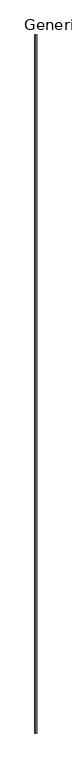
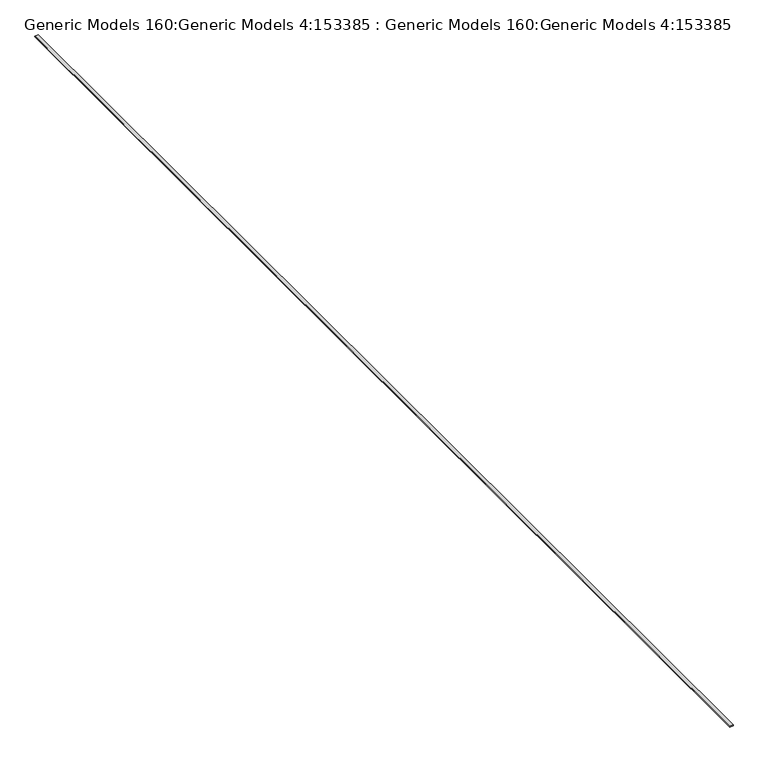
"""IFC4 building model written with IfcOpenShell, lengths in millimetres: proxy geometry, Generic Models 160:Generic Models 4:153385 : Generic Models 160:Generic Models 4:153385."""

from ifc_helpers import new_model, si_unit, point, frame, frame_2d, origin, place, context, project, spatial, polyline, circle_curve, trimmed, segment, composite_curve, outline, extrude, source, transform, mapped, element, save


def generic_models_160_generic_models_4_153385_generic_models_e2b97bb7(model_context):
    return source(origin(), model_context, "Body", "SweptSolid", [
        extrude(outline(composite_curve([segment(polyline([(-503.9725126, -10294.1571126), (-503.9725126, -10331.3078813)]), True, "CONTINUOUS"), segment(trimmed(circle_curve(frame_2d((-508.7350126, -10333.721994)), 5.3394144), [point((-503.9725126, -10331.3078813))], [point((-513.4975126, -10331.3078813))], True, "CARTESIAN"), True, "CONTINUOUS"), segment(polyline([(-513.4975126, -10331.3078813), (-513.4975126, -10294.1571126), (-503.9725126, -10294.1571126)]), True, "CONTINUOUS")], self_intersect=False)), frame((0.0, -5303.1974793, 0.0), z_axis=(0.0, 1.0, 0.0), x_axis=(0.0, 0.0, 1.0)), (0.0, 0.0, 1.0), 12547.6),
    ])


if __name__ == "__main__":
    model = new_model("IFC4")
    model_context = context("Model", 3, world=origin())
    ifc_project = project(units=[si_unit("LENGTHUNIT", "METRE", prefix="MILLI")], contexts=[model_context])
    site = spatial("IfcSite", under=ifc_project)
    building = spatial("IfcBuilding", under=site)
    placement = place(None, origin())
    generic_models_160_generic_models_4_153385_generic_models_shape = generic_models_160_generic_models_4_153385_generic_models_e2b97bb7(model_context)
    element("IfcBuildingElementProxy", 1, Name="Generic Models 160:Generic Models 4:153385 : Generic Models 160:Generic Models 4:153385", ObjectType="Generic Models 160:Generic Models 4:153385 : Generic Models 160:Generic Models 4:153385", at=placement, inside=building, context=model_context, shape_type="MappedRepresentation", body=[
        mapped(generic_models_160_generic_models_4_153385_generic_models_shape, transform((0.0, 0.0, 0.0), x_axis=(1.0, 0.0, 0.0), y_axis=(0.0, 1.0, 0.0), z_axis=(0.0, 0.0, 1.0))),
    ])
    save(model, "model.ifc")

# Revit data of these elements
# Type "Generic Models 160:Generic Models 4:153385 : Generic Models 160:Generic Models 4:153385"
#   NameOverride = "Generic Models 160:Generic Models 4:153385"
#   ObjectTypeOverride = "Generic Models 160:Generic Models 4"
#   Reference = "Generic Models 4"
#   Category = "Generic Models"
#   Tag = "153385"
# Element 1 (IfcBuildingElementProxy, "Generic Models 160:Generic Models 4:153385 : Generic Models 160:Generic Models 4:153385")
#   Materials on its faces: "_MORTAR SETTING BED 12838"
# Materials
#   "_MORTAR SETTING BED 12838": class "Unassigned", colour RGB 191 191 191, transparency 0
